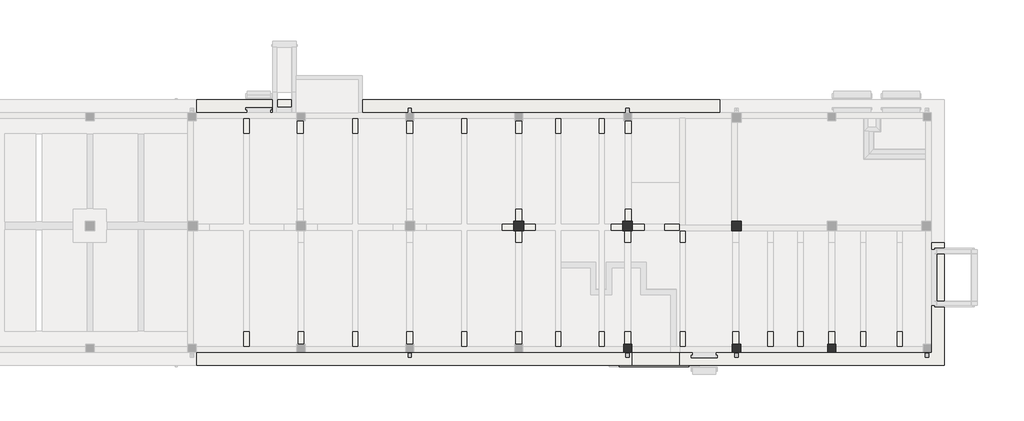
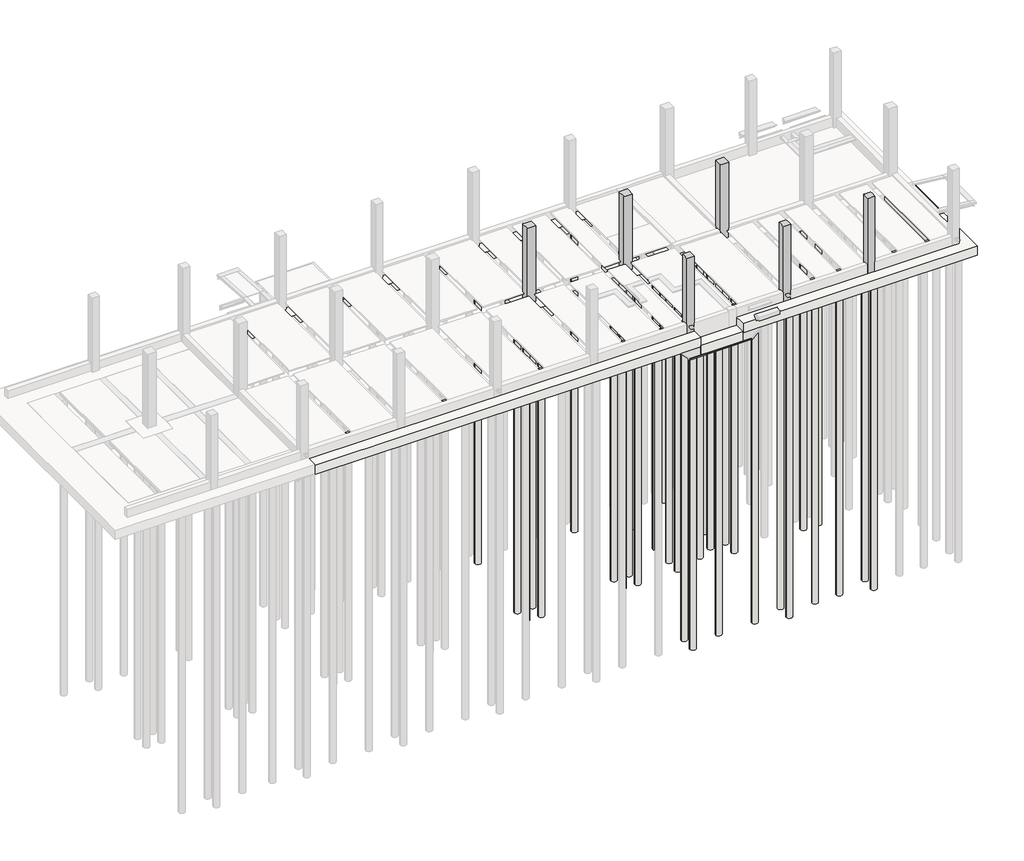
# One storey, part 5 of 7: 42 slabs, 6 columns.
"""IFC4 building model written with IfcOpenShell, lengths in millimetres."""

from ifc_helpers import new_model, si_unit, point, frame, frame_2d, origin, place, context, project, spatial, polyline, circle_curve, trimmed, segment, composite_curve, outline, extrude, faceted_brep, element, save

model = new_model("IFC4")

# Units and contexts
model_context = context("Model", 3, world=origin())
ifc_project = project(units=[si_unit("LENGTHUNIT", "METRE", prefix="MILLI")], contexts=[model_context])

# Site, building, storey
site = spatial("IfcSite", under=ifc_project)
building = spatial("IfcBuilding", under=site)
storey = spatial("IfcBuildingStorey", under=building, Name="H.P.P", Elevation=4500.0)

# Columns
placement = place(None, origin())
element("IfcColumn", 1, ObjectType="RC_Column_Rectangular : H_SC_AR S15_RC Col-AG_700x700_C1", at=placement, inside=storey, context=model_context, shape_type="Brep", body=[
    faceted_brep([(39350.0000001, -7650.0, 4000.0), (39350.0000001, -8350.0, 4000.0), (38650.0000001, -8350.0, 4000.0), (38650.0000001, -7650.0, 4000.0), (39350.0000001, -7650.0, 4650.0), (39350.0000001, -7650.0, 4800.0), (39350.0000001, -7650.0, 10450.0), (39350.0000001, -7650.0, 10600.0), (39350.0000001, -7700.0, 10600.0), (39350.0000001, -8300.0, 10600.0), (39350.0000001, -8350.0, 10600.0), (39350.0000001, -8350.0, 10450.0), (39350.0000001, -8350.0, 4800.0), (39350.0000001, -8350.0, 4650.0), (39249.9999998, -8350.0, 10600.0), (38750.0000002, -8350.0, 10600.0), (38650.0000001, -8350.0, 10600.0), (38650.0000001, -8350.0, 10450.0), (38650.0000001, -8350.0, 4800.0), (38650.0000001, -8350.0, 4650.0), (38650.0000001, -8300.0, 10600.0), (38650.0000001, -7700.0, 10600.0), (38650.0000001, -7650.0, 10600.0), (38650.0000001, -7650.0, 10450.0), (38650.0000001, -7650.0, 4800.0), (38650.0000001, -7650.0, 4650.0), (38750.0000002, -7650.0, 10600.0), (39249.9999998, -7650.0, 10600.0)], [[[0, 1, 2, 3]], [[1, 0, 4, 5, 6, 7, 8, 9, 10, 11, 12, 13]], [[2, 1, 13, 12, 11, 10, 14, 15, 16, 17, 18, 19]], [[3, 2, 19, 18, 17, 16, 20, 21, 22, 23, 24, 25]], [[0, 3, 25, 24, 23, 22, 26, 27, 7, 6, 5, 4]], [[8, 7, 27, 26, 22, 21, 20, 16, 15, 14, 10, 9]]]),
])
element("IfcColumn", 2, ObjectType="RC_Column_Rectangular : H_SC_AR S15_RC Col-AG_700x700_C1", at=placement, inside=storey, context=model_context, shape_type="Brep", body=[
    faceted_brep([(47349.9999999, -7650.0, 4000.0), (47349.9999999, -8350.0, 4000.0), (47250.0, -8350.0, 4000.0), (46750.0, -8350.0, 4000.0), (46649.9999999, -8350.0, 4000.0), (46649.9999999, -7650.0, 4000.0), (47349.9999999, -7650.0, 4650.0), (47349.9999999, -7850.0, 4650.0), (47349.9999999, -7850.0, 4800.0), (47349.9999999, -7650.0, 4800.0), (47349.9999999, -7650.0, 10450.0), (47349.9999999, -7650.0, 10600.0), (47349.9999999, -7750.0, 10600.0), (47349.9999999, -8350.0, 10600.0), (47349.9999999, -8350.0, 10450.0), (47349.9999999, -8350.0, 4800.0), (47349.9999999, -8350.0, 4650.0), (47300.0, -8350.0, 10600.0), (46800.0, -8350.0, 10600.0), (46649.9999999, -8350.0, 10600.0), (46649.9999999, -8350.0, 10450.0), (46649.9999999, -8350.0, 4800.0), (46649.9999999, -8350.0, 4650.0), (46649.9999999, -8300.0, 10600.0), (46649.9999999, -7700.0, 10600.0), (46649.9999999, -7650.0, 10600.0), (46649.9999999, -7650.0, 10450.0), (46649.9999999, -7650.0, 4800.0), (46649.9999999, -7650.0, 4650.0), (46800.0, -7650.0, 10600.0), (47300.0, -7650.0, 10600.0), (47300.0, -7650.0, 4800.0), (47300.0, -7650.0, 4650.0), (47300.0, -7850.0, 4650.0), (47300.0, -7850.0, 4800.0)], [[[0, 1, 2, 3, 4, 5]], [[1, 0, 6, 7, 8, 9, 10, 11, 12, 13, 14, 15, 16]], [[4, 3, 2, 1, 16, 15, 14, 13, 17, 18, 19, 20, 21, 22]], [[5, 4, 22, 21, 20, 19, 23, 24, 25, 26, 27, 28]], [[0, 5, 28, 27, 26, 25, 29, 30, 11, 10, 9, 31, 32, 6]], [[12, 11, 30, 29, 25, 24, 23, 19, 18, 17, 13]], [[32, 33, 7, 6]], [[8, 34, 31, 9]], [[33, 34, 8, 7]], [[34, 33, 32, 31]]]),
])
element("IfcColumn", 3, ObjectType="RC_Column_Rectangular : H_SC_AR S15_RC Col-AG_700x700_C1", at=placement, inside=storey, context=model_context, shape_type="Brep", body=[
    faceted_brep([(55350.0, -7650.0, 4000.0), (55350.0, -7950.0, 4000.0), (55350.0, -8350.0, 4000.0), (54650.0, -8350.0, 4000.0), (54650.0, -7950.0, 4000.0), (54650.0, -7650.0, 4000.0), (55050.0, -7650.0, 4000.0), (55350.0, -7650.0, 10600.0), (55350.0, -8350.0, 10600.0), (55350.0, -8350.0, 10450.0), (55350.0, -8350.0, 9800.0), (55350.0, -8350.0, 4800.0), (55350.0, -8350.0, 4650.0), (55200.0, -8350.0, 10600.0), (54700.0, -8350.0, 10600.0), (54650.0, -8350.0, 10600.0), (54650.0, -8350.0, 10450.0), (54650.0, -8350.0, 9700.0), (54650.0, -8350.0, 4800.0), (54650.0, -8350.0, 4650.0), (54650.0, -7650.0, 10600.0), (54650.0, -7650.0, 9800.0), (54650.0, -7650.0, 4800.0)], [[[0, 1, 2, 3, 4, 5, 6]], [[2, 1, 0, 7, 8, 9, 10, 11, 12]], [[3, 2, 12, 11, 10, 9, 8, 13, 14, 15, 16, 17, 18, 19]], [[5, 4, 3, 19, 18, 17, 16, 15, 20, 21, 22]], [[0, 6, 5, 22, 21, 20, 7]], [[8, 7, 20, 15, 14, 13]]]),
])
element("IfcColumn", 4, ObjectType="RC_Column_Rectangular : H_SC_AR S15_RC Col-AG_600x600_C2", at=placement, inside=storey, context=model_context, shape_type="Brep", body=[
    faceted_brep([(62300.0, -16700.0, 4000.0), (62300.0, -16900.0, 4000.0), (62300.0, -17300.0, 4000.0), (61700.0, -17300.0, 4000.0), (61700.0, -16900.0, 4000.0), (61700.0, -16700.0, 4000.0), (62300.0, -16700.0, 4650.0), (62300.0, -16700.0, 4800.0), (62300.0, -16700.0, 10450.0), (62300.0, -16700.0, 10600.0), (62300.0, -16900.0, 10600.0), (62300.0, -17300.0, 10600.0), (62300.0, -17300.0, 9800.0), (62300.0, -17300.0, 4800.0), (61700.0, -17300.0, 10600.0), (61700.0, -17300.0, 9800.0), (61700.0, -17300.0, 4800.0), (61700.0, -16900.0, 10600.0), (61700.0, -16700.0, 10600.0), (61700.0, -16700.0, 10450.0), (61700.0, -16700.0, 4800.0), (61700.0, -16700.0, 4650.0), (61750.0, -16700.0, 10600.0), (62250.0, -16700.0, 10600.0)], [[[0, 1, 2, 3, 4, 5]], [[2, 1, 0, 6, 7, 8, 9, 10, 11, 12, 13]], [[3, 2, 13, 12, 11, 14, 15, 16]], [[5, 4, 3, 16, 15, 14, 17, 18, 19, 20, 21]], [[0, 5, 21, 20, 19, 18, 22, 23, 9, 8, 7, 6]], [[14, 11, 10, 9, 23, 22, 18, 17]]]),
])
element("IfcColumn", 5, ObjectType="RC_Column_Rectangular : H_SC_AR S15_RC Col-AG_600x600_C2", at=placement, inside=storey, context=model_context, shape_type="Brep", body=[
    faceted_brep([(55300.0, -16700.0, 4000.0), (55300.0, -16900.0, 4000.0), (55300.0, -17300.0, 4000.0), (54700.0, -17300.0, 4000.0), (54700.0, -16900.0, 4000.0), (54700.0, -16700.0, 4000.0), (55300.0, -16700.0, 4650.0), (55300.0, -16700.0, 4800.0), (55300.0, -16700.0, 10450.0), (55300.0, -16700.0, 10600.0), (55300.0, -16900.0, 10600.0), (55300.0, -17300.0, 10600.0), (55300.0, -17300.0, 9800.0), (55300.0, -17300.0, 4800.0), (54700.0, -17300.0, 10600.0), (54700.0, -17300.0, 9800.0), (54700.0, -17300.0, 4800.0), (54700.0, -16900.0, 10600.0), (54700.0, -16700.0, 10600.0), (54700.0, -16700.0, 10450.0), (54700.0, -16700.0, 4800.0), (54700.0, -16700.0, 4650.0), (55200.0, -16700.0, 10600.0)], [[[0, 1, 2, 3, 4, 5]], [[2, 1, 0, 6, 7, 8, 9, 10, 11, 12, 13]], [[3, 2, 13, 12, 11, 14, 15, 16]], [[5, 4, 3, 16, 15, 14, 17, 18, 19, 20, 21]], [[0, 5, 21, 20, 19, 18, 22, 9, 8, 7, 6]], [[14, 11, 10, 9, 22, 18, 17]]]),
])
element("IfcColumn", 6, ObjectType="RC_Column_Rectangular : H_SC_AR S15_RC Col-AG_600x600_C2", at=placement, inside=storey, context=model_context, shape_type="Brep", body=[
    faceted_brep([(46700.0, -16700.0, 4000.0), (47300.0, -16700.0, 4000.0), (47300.0, -17300.0, 4000.0), (46700.0, -17300.0, 4000.0), (46700.0, -16900.0, 4000.0), (46700.0, -16700.0, 4550.0), (46700.0, -16700.0, 4700.0), (46700.0, -16700.0, 10450.0), (46700.0, -16700.0, 10600.0), (46800.0, -16700.0, 10600.0), (47300.0, -16700.0, 10600.0), (47300.0, -16700.0, 10450.0), (47300.0, -16700.0, 4700.0), (47300.0, -16700.0, 4550.0), (47300.0, -16900.0, 10600.0), (47300.0, -17300.0, 10600.0), (47300.0, -17300.0, 9800.0), (47300.0, -17300.0, 4700.0), (46700.0, -17300.0, 10600.0), (46700.0, -17300.0, 9800.0), (46700.0, -17300.0, 4800.0), (46700.0, -16900.0, 10600.0)], [[[0, 1, 2, 3, 4]], [[1, 0, 5, 6, 7, 8, 9, 10, 11, 12, 13]], [[2, 1, 13, 12, 11, 10, 14, 15, 16, 17]], [[3, 2, 17, 16, 15, 18, 19, 20]], [[0, 4, 3, 20, 19, 18, 21, 8, 7, 6, 5]], [[18, 15, 14, 10, 9, 8, 21]]]),
])

# Slabs
element("IfcSlab", 7, ObjectType="H_SF_AR S18_MAT_T800_WF1", at=placement, inside=storey, context=model_context, shape_type="Brep", body=[
    faceted_brep([(50825.0, -18250.0000001, 3200.0), (50825.0, -15750.0000001, 3200.0), (52225.0, -15750.0000001, 3200.0), (67750.0000002, -15750.0000001, 3200.0), (67750.0000002, -9250.0, 3200.0), (70250.0, -9250.0, 3200.0), (70250.0, -18250.0000001, 3200.0), (52225.0, -18250.0000001, 3200.0), (50825.0, -18250.0000001, 4000.0), (70250.0, -18250.0000001, 4000.0), (70250.0, -9250.0, 4000.0), (67750.0000002, -9250.0, 4000.0), (67750.0000002, -15750.0000001, 4000.0), (50825.0, -15750.0000001, 4000.0), (50825.0, -16900.0, 4000.0), (50825.0, -18250.0000001, 3300.0), (50825.0, -15750.0000001, 3300.0)], [[[0, 1, 2, 3, 4, 5, 6, 7]], [[8, 9, 10, 11, 12, 13, 14]], [[6, 5, 10, 9]], [[0, 7, 6, 9, 8, 15]], [[3, 2, 1, 16, 13, 12]], [[4, 3, 12, 11]], [[1, 0, 15, 8, 14, 13, 16]], [[5, 4, 11, 10]]]),
    faceted_brep([(15299.9999999, -18250.0000001, 3200.0), (15299.9999999, -15750.0000001, 3200.0), (45675.0, -15750.0000001, 3200.0), (47300.0, -15750.0000001, 3200.0), (47300.0, -18250.0000001, 3200.0), (45675.0, -18250.0000001, 3200.0), (15299.9999999, -18250.0000001, 4000.0), (47300.0, -18250.0000001, 4000.0), (47300.0, -15750.0000001, 4000.0), (15299.9999999, -15750.0000001, 4000.0), (15299.9999999, -18250.0000001, 3300.0), (15299.9999999, -15750.0000001, 3300.0), (47300.0, -15750.0000001, 3300.0), (47300.0, -18250.0000001, 3300.0)], [[[0, 1, 2, 3, 4, 5]], [[6, 7, 8, 9]], [[1, 0, 10, 6, 9, 11]], [[3, 2, 1, 11, 9, 8, 12]], [[4, 3, 12, 8, 7, 13]], [[0, 5, 4, 13, 7, 6, 10]]]),
    faceted_brep([(53749.9998007, 1249.9999999, 3200.0), (53749.9998007, -1250.0000001, 3200.0), (52200.0000002, -1250.0000001, 3200.0), (52200.0000002, -6750.0000001, 3200.0), (53749.9998007, -6750.0000001, 3200.0), (53749.9998007, -9250.0, 3200.0), (49700.0000002, -9250.0, 3200.0), (49700.0000002, -1250.0000001, 3200.0), (15299.9999999, -1250.0000001, 3200.0), (15299.9999999, 1249.9999999, 3200.0), (53749.9998007, 1249.9999999, 4000.0), (15299.9999999, 1249.9999999, 4000.0), (15299.9999999, -1250.0000001, 4000.0), (49700.0000002, -1250.0000001, 4000.0), (49700.0000002, -9250.0, 4000.0), (53749.9998007, -9250.0, 4000.0), (53749.9998007, -6750.0000001, 4000.0), (52200.0000002, -6750.0000001, 4000.0), (52200.0000002, -1250.0000001, 4000.0), (53749.9998007, -1250.0000001, 4000.0), (15299.9999999, 1249.9999999, 3300.0), (15299.9999999, -1250.0000001, 3300.0)], [[[0, 1, 2, 3, 4, 5, 6, 7, 8, 9]], [[10, 11, 12, 13, 14, 15, 16, 17, 18, 19]], [[0, 9, 20, 11, 10]], [[6, 5, 15, 14]], [[7, 6, 14, 13]], [[8, 7, 13, 12, 21]], [[2, 1, 19, 18]], [[3, 2, 18, 17]], [[4, 3, 17, 16]], [[1, 0, 10, 19]], [[9, 8, 21, 12, 11, 20]], [[5, 4, 16, 15]]]),
])
element("IfcSlab", 8, ObjectType="H_SF_AR S18_MAT_T800_WF1", at=placement, inside=storey, context=model_context, shape_type="Brep", body=[
    faceted_brep([(50825.0, -15750.0000001, 2500.0), (50825.0, -18250.0000001, 2500.0), (47300.0, -18250.0000001, 2500.0), (47300.0, -15750.0000001, 2500.0), (50825.0, -18250.0000001, 3300.0), (50825.0, -15750.0000001, 3300.0), (47300.0, -15750.0000001, 3300.0), (47300.0, -18250.0000001, 3300.0), (50825.0, -15750.0000001, 3200.0), (50825.0, -18250.0000001, 3200.0), (47300.0, -18250.0000001, 3200.0), (47300.0, -15750.0000001, 3200.0)], [[[0, 1, 2, 3]], [[4, 5, 6, 7]], [[1, 0, 8, 5, 4, 9]], [[2, 1, 9, 4, 7, 10]], [[3, 2, 10, 7, 6, 11]], [[0, 3, 11, 6, 5, 8]]]),
])
element("IfcSlab", 9, ObjectType="H_SF_AR_S18_Lean_T50", at=placement, inside=storey, context=model_context, shape_type="SweptSolid", body=[
    extrude(outline(polyline([(51525.0, -15650.0), (51525.0, -18350.0000001), (46375.0, -18350.0000001), (46375.0, -15650.0), (51525.0, -15650.0)])), frame((0.0, 0.0, 2450.0), z_axis=(0.0, 0.0, 1.0), x_axis=(1.0, 0.0, 0.0)), (0.0, 0.0, 1.0), 50.0),
])
element("IfcSlab", 10, ObjectType="H_SF_AR_S18_Lean_T50", at=placement, inside=storey, context=model_context, shape_type="Brep", body=[
    faceted_brep([(50475.0, -16790.0, 4390.0), (47360.0, -16790.0, 4390.0), (47360.0, -10775.0, 4390.0), (48275.0, -10775.0, 4390.0), (48275.0, -12775.0, 4390.0), (50475.0, -12775.0, 4390.0), (47360.0, -16790.0, 4440.0), (50475.0, -16790.0, 4440.0), (50475.0, -12775.0, 4440.0), (48275.0, -12775.0, 4440.0), (48275.0, -10775.0, 4440.0), (47360.0, -10775.0, 4440.0)], [[[0, 1, 2, 3, 4, 5]], [[6, 7, 8, 9, 10, 11]], [[1, 0, 7, 6]], [[2, 1, 6, 11]], [[3, 2, 11, 10]], [[4, 3, 10, 9]], [[5, 4, 9, 8]], [[0, 5, 8, 7]]]),
    faceted_brep([(46640.0, -10775.0, 4390.0), (46640.0, -16790.0, 4390.0), (45435.0, -16790.0, 4390.0), (45435.0, -12775.0, 4390.0), (45504.2893219, -12775.0, 4390.0), (45525.0, -12775.0, 4390.0), (45525.0, -10775.0, 4390.0), (46640.0, -16790.0, 4440.0), (46640.0, -10775.0, 4440.0), (45525.0, -10775.0, 4440.0), (45525.0, -12775.0, 4440.0), (45454.2893219, -12775.0, 4440.0), (45435.0, -12775.0, 4440.0), (45435.0, -16790.0, 4440.0)], [[[0, 1, 2, 3, 4, 5, 6]], [[7, 8, 9, 10, 11, 12, 13]], [[1, 0, 8, 7]], [[2, 1, 7, 13]], [[3, 2, 13, 12]], [[3, 12, 11, 10, 5, 4]], [[6, 5, 10, 9]], [[0, 6, 9, 8]]]),
    faceted_brep([(44765.0, -12775.0, 4390.0), (44765.0, -16790.0, 4390.0), (42235.0, -16790.0, 4390.0), (42235.0, -10775.0, 4390.0), (44575.0, -10775.0, 4390.0), (44575.0, -12775.0, 4390.0), (44765.0, -16790.0, 4440.0), (44765.0, -12775.0, 4440.0), (44575.0, -12775.0, 4440.0), (44575.0, -10775.0, 4440.0), (42235.0, -10775.0, 4440.0), (42235.0, -16790.0, 4440.0)], [[[0, 1, 2, 3, 4, 5]], [[6, 7, 8, 9, 10, 11]], [[1, 0, 7, 6]], [[2, 1, 6, 11]], [[3, 2, 11, 10]], [[4, 3, 10, 9]], [[5, 4, 9, 8]], [[0, 5, 8, 7]]]),
    faceted_brep([(47410.0, -4825.0, 4390.0), (47410.0, -210.0, 4390.0), (50825.0, -210.0, 4390.0), (50825.0, -4825.0, 4390.0), (47410.0, -210.0, 4440.0), (47410.0, -4825.0, 4440.0), (50825.0, -4825.0, 4440.0), (50825.0, -210.0, 4440.0)], [[[0, 1, 2, 3]], [[4, 5, 6, 7]], [[1, 0, 5, 4]], [[2, 1, 4, 7]], [[3, 2, 7, 6]], [[0, 3, 6, 5]]]),
])
element("IfcSlab", 11, ObjectType="H_SF_AR_S18_Lean_T50", at=placement, inside=storey, context=model_context, shape_type="SweptSolid", body=[
    extrude(outline(polyline([(54650.0, -100.0), (54650.0, -7950.0), (51225.0, -7950.0), (51225.0, -100.0), (54650.0, -100.0)])), frame((0.0, 0.0, 4440.0), z_axis=(0.0, 0.0, 1.0), x_axis=(1.0, 0.0, 0.0)), (0.0, 0.0, 1.0), 50.0),
])
element("IfcSlab", 12, ObjectType="Foundation Rectangular (Non-Pile) : H_SF_AR S18_Ret Fdn_2500x2500xT1000_F1A", at=placement, inside=storey, context=model_context, shape_type="SweptSolid", body=[
    extrude(outline(polyline([(40250.0000001, -6750.0), (40250.0000001, -9250.0), (37750.0000001, -9250.0), (37750.0000001, -6750.0), (40250.0000001, -6750.0)])), frame((0.0, 0.0, 3000.0), z_axis=(0.0, 0.0, 1.0), x_axis=(1.0, 0.0, 0.0)), (0.0, 0.0, 1.0), 1000.0),
])
element("IfcSlab", 13, ObjectType="Foundation Rectangular (Non-Pile) : H_SF_AR S18_Ret Fdn_2500x2500xT1000_F1A", at=placement, inside=storey, context=model_context, shape_type="SweptSolid", body=[
    extrude(outline(polyline([(48249.9999999, -6750.0), (48249.9999999, -9250.0), (45749.9999999, -9250.0), (45749.9999999, -6750.0), (48249.9999999, -6750.0)])), frame((0.0, 0.0, 3000.0), z_axis=(0.0, 0.0, 1.0), x_axis=(1.0, 0.0, 0.0)), (0.0, 0.0, 1.0), 1000.0),
])
element("IfcSlab", 14, ObjectType="PILE : H_FL_AR S19_Pile_D500_L26.8", at=placement, inside=storey, context=model_context, shape_type="SweptSolid", body=[
    extrude(outline(composite_curve([segment(trimmed(circle_curve(frame_2d((39000.0, -625.0)), 250.0), [point((38750.0, -625.0))], [point((39250.0, -625.0))], False, "CARTESIAN"), True, "CONTINUOUS"), segment(trimmed(circle_curve(frame_2d((39000.0, -625.0)), 250.0), [point((39250.0, -625.0))], [point((38750.0, -625.0))], False, "CARTESIAN"), True, "CONTINUOUS")], self_intersect=False)), frame((0.0, 0.0, -23500.0), z_axis=(0.0, 0.0, 1.0), x_axis=(1.0, 0.0, 0.0)), (0.0, 0.0, 1.0), 26650.0),
])
element("IfcSlab", 15, ObjectType="PILE : H_FL_AR S19_Pile_D500_L26.8", at=placement, inside=storey, context=model_context, shape_type="SweptSolid", body=[
    extrude(outline(composite_curve([segment(trimmed(circle_curve(frame_2d((47000.0, -625.0000002)), 250.0), [point((46750.0, -625.0000002))], [point((47250.0, -625.0000002))], False, "CARTESIAN"), True, "CONTINUOUS"), segment(trimmed(circle_curve(frame_2d((47000.0, -625.0000002)), 250.0), [point((47250.0, -625.0000002))], [point((46750.0, -625.0000002))], False, "CARTESIAN"), True, "CONTINUOUS")], self_intersect=False)), frame((0.0, 0.0, -23500.0), z_axis=(0.0, 0.0, 1.0), x_axis=(1.0, 0.0, 0.0)), (0.0, 0.0, 1.0), 26650.0),
])
element("IfcSlab", 16, ObjectType="PILE : H_FL_AR S19_Pile_D500_L26.8", at=placement, inside=storey, context=model_context, shape_type="SweptSolid", body=[
    extrude(outline(composite_curve([segment(trimmed(circle_curve(frame_2d((50950.0000002, -625.0)), 250.0), [point((50700.0000002, -625.0))], [point((51200.0000002, -625.0))], False, "CARTESIAN"), True, "CONTINUOUS"), segment(trimmed(circle_curve(frame_2d((50950.0000002, -625.0)), 250.0), [point((51200.0000002, -625.0))], [point((50700.0000002, -625.0))], False, "CARTESIAN"), True, "CONTINUOUS")], self_intersect=False)), frame((0.0, 0.0, -23500.0), z_axis=(0.0, 0.0, 1.0), x_axis=(1.0, 0.0, 0.0)), (0.0, 0.0, 1.0), 26650.0),
])
element("IfcSlab", 17, ObjectType="PILE : H_FL_AR S19_Pile_D500_L26.8", at=placement, inside=storey, context=model_context, shape_type="SweptSolid", body=[
    extrude(outline(composite_curve([segment(trimmed(circle_curve(frame_2d((50950.0000002, -2500.0)), 250.0), [point((50700.0000002, -2500.0))], [point((51200.0000002, -2500.0))], False, "CARTESIAN"), True, "CONTINUOUS"), segment(trimmed(circle_curve(frame_2d((50950.0000002, -2500.0)), 250.0), [point((51200.0000002, -2500.0))], [point((50700.0000002, -2500.0))], False, "CARTESIAN"), True, "CONTINUOUS")], self_intersect=False)), frame((0.0, 0.0, -23500.0), z_axis=(0.0, 0.0, 1.0), x_axis=(1.0, 0.0, 0.0)), (0.0, 0.0, 1.0), 26650.0),
])
element("IfcSlab", 18, ObjectType="PILE : H_FL_AR S19_Pile_D500_L26.8", at=placement, inside=storey, context=model_context, shape_type="SweptSolid", body=[
    extrude(outline(composite_curve([segment(trimmed(circle_curve(frame_2d((50950.0000002, -5500.0)), 250.0), [point((50700.0000002, -5500.0))], [point((51200.0000002, -5500.0))], False, "CARTESIAN"), True, "CONTINUOUS"), segment(trimmed(circle_curve(frame_2d((50950.0000002, -5500.0)), 250.0), [point((51200.0000002, -5500.0))], [point((50700.0000002, -5500.0))], False, "CARTESIAN"), True, "CONTINUOUS")], self_intersect=False)), frame((0.0, 0.0, -23500.0), z_axis=(0.0, 0.0, 1.0), x_axis=(1.0, 0.0, 0.0)), (0.0, 0.0, 1.0), 26650.0),
])
element("IfcSlab", 19, ObjectType="PILE : H_FL_AR S19_Pile_D500_L26.8", at=placement, inside=storey, context=model_context, shape_type="SweptSolid", body=[
    extrude(outline(composite_curve([segment(trimmed(circle_curve(frame_2d((50950.0000002, -7375.0000222)), 250.0), [point((50700.0000002, -7375.0000222))], [point((51200.0000002, -7375.0000222))], False, "CARTESIAN"), True, "CONTINUOUS"), segment(trimmed(circle_curve(frame_2d((50950.0000002, -7375.0000222)), 250.0), [point((51200.0000002, -7375.0000222))], [point((50700.0000002, -7375.0000222))], False, "CARTESIAN"), True, "CONTINUOUS")], self_intersect=False)), frame((0.0, 0.0, -23500.0), z_axis=(0.0, 0.0, 1.0), x_axis=(1.0, 0.0, 0.0)), (0.0, 0.0, 1.0), 26650.0),
])
element("IfcSlab", 20, ObjectType="PILE : H_FL_AR S19_Pile_D500_L26.8", at=placement, inside=storey, context=model_context, shape_type="SweptSolid", body=[
    extrude(outline(composite_curve([segment(trimmed(circle_curve(frame_2d((50950.0000002, -8625.0000222)), 250.0), [point((50700.0000002, -8625.0000222))], [point((51200.0000002, -8625.0000222))], False, "CARTESIAN"), True, "CONTINUOUS"), segment(trimmed(circle_curve(frame_2d((50950.0000002, -8625.0000222)), 250.0), [point((51200.0000002, -8625.0000222))], [point((50700.0000002, -8625.0000222))], False, "CARTESIAN"), True, "CONTINUOUS")], self_intersect=False)), frame((0.0, 0.0, -23500.0), z_axis=(0.0, 0.0, 1.0), x_axis=(1.0, 0.0, 0.0)), (0.0, 0.0, 1.0), 26650.0),
])
element("IfcSlab", 21, ObjectType="PILE : H_FL_AR S19_Pile_D500_L26.8", at=placement, inside=storey, context=model_context, shape_type="SweptSolid", body=[
    extrude(outline(composite_curve([segment(trimmed(circle_curve(frame_2d((53125.0, -8000.0)), 250.0), [point((52875.0, -8000.0))], [point((53375.0, -8000.0))], False, "CARTESIAN"), True, "CONTINUOUS"), segment(trimmed(circle_curve(frame_2d((53125.0, -8000.0)), 250.0), [point((53375.0, -8000.0))], [point((52875.0, -8000.0))], False, "CARTESIAN"), True, "CONTINUOUS")], self_intersect=False)), frame((0.0, 0.0, -23500.0), z_axis=(0.0, 0.0, 1.0), x_axis=(1.0, 0.0, 0.0)), (0.0, 0.0, 1.0), 26650.0),
])
element("IfcSlab", 22, ObjectType="PILE : H_FL_AR S19_Pile_D500_L26.6", at=placement, inside=storey, context=model_context, shape_type="SweptSolid", body=[
    extrude(outline(composite_curve([segment(trimmed(circle_curve(frame_2d((38375.0000004, -7374.9999999)), 250.0), [point((38125.0000004, -7374.9999999))], [point((38625.0000004, -7374.9999999))], False, "CARTESIAN"), True, "CONTINUOUS"), segment(trimmed(circle_curve(frame_2d((38375.0000004, -7374.9999999)), 250.0), [point((38625.0000004, -7374.9999999))], [point((38125.0000004, -7374.9999999))], False, "CARTESIAN"), True, "CONTINUOUS")], self_intersect=False)), frame((0.0, 0.0, -23500.0), z_axis=(0.0, 0.0, 1.0), x_axis=(1.0, 0.0, 0.0)), (0.0, 0.0, 1.0), 26450.0),
])
element("IfcSlab", 23, ObjectType="PILE : H_FL_AR S19_Pile_D500_L26.6", at=placement, inside=storey, context=model_context, shape_type="SweptSolid", body=[
    extrude(outline(composite_curve([segment(trimmed(circle_curve(frame_2d((39625.0000004, -7374.9999999)), 250.0), [point((39375.0000004, -7374.9999999))], [point((39875.0000004, -7374.9999999))], False, "CARTESIAN"), True, "CONTINUOUS"), segment(trimmed(circle_curve(frame_2d((39625.0000004, -7374.9999999)), 250.0), [point((39875.0000004, -7374.9999999))], [point((39375.0000004, -7374.9999999))], False, "CARTESIAN"), True, "CONTINUOUS")], self_intersect=False)), frame((0.0, 0.0, -23500.0), z_axis=(0.0, 0.0, 1.0), x_axis=(1.0, 0.0, 0.0)), (0.0, 0.0, 1.0), 26450.0),
])
element("IfcSlab", 24, ObjectType="PILE : H_FL_AR S19_Pile_D500_L26.6", at=placement, inside=storey, context=model_context, shape_type="SweptSolid", body=[
    extrude(outline(composite_curve([segment(trimmed(circle_curve(frame_2d((38375.0000004, -8624.9999999)), 250.0), [point((38125.0000004, -8624.9999999))], [point((38625.0000004, -8624.9999999))], False, "CARTESIAN"), True, "CONTINUOUS"), segment(trimmed(circle_curve(frame_2d((38375.0000004, -8624.9999999)), 250.0), [point((38625.0000004, -8624.9999999))], [point((38125.0000004, -8624.9999999))], False, "CARTESIAN"), True, "CONTINUOUS")], self_intersect=False)), frame((0.0, 0.0, -23500.0), z_axis=(0.0, 0.0, 1.0), x_axis=(1.0, 0.0, 0.0)), (0.0, 0.0, 1.0), 26450.0),
])
element("IfcSlab", 25, ObjectType="PILE : H_FL_AR S19_Pile_D500_L26.6", at=placement, inside=storey, context=model_context, shape_type="SweptSolid", body=[
    extrude(outline(composite_curve([segment(trimmed(circle_curve(frame_2d((39625.0000004, -8624.9999999)), 250.0), [point((39375.0000004, -8624.9999999))], [point((39875.0000004, -8624.9999999))], False, "CARTESIAN"), True, "CONTINUOUS"), segment(trimmed(circle_curve(frame_2d((39625.0000004, -8624.9999999)), 250.0), [point((39875.0000004, -8624.9999999))], [point((39375.0000004, -8624.9999999))], False, "CARTESIAN"), True, "CONTINUOUS")], self_intersect=False)), frame((0.0, 0.0, -23500.0), z_axis=(0.0, 0.0, 1.0), x_axis=(1.0, 0.0, 0.0)), (0.0, 0.0, 1.0), 26450.0),
])
element("IfcSlab", 26, ObjectType="PILE : H_FL_AR S19_Pile_D500_L26.6", at=placement, inside=storey, context=model_context, shape_type="SweptSolid", body=[
    extrude(outline(composite_curve([segment(trimmed(circle_curve(frame_2d((46375.0000004, -7374.9999999)), 250.0), [point((46125.0000004, -7374.9999999))], [point((46625.0000004, -7374.9999999))], False, "CARTESIAN"), True, "CONTINUOUS"), segment(trimmed(circle_curve(frame_2d((46375.0000004, -7374.9999999)), 250.0), [point((46625.0000004, -7374.9999999))], [point((46125.0000004, -7374.9999999))], False, "CARTESIAN"), True, "CONTINUOUS")], self_intersect=False)), frame((0.0, 0.0, -23500.0), z_axis=(0.0, 0.0, 1.0), x_axis=(1.0, 0.0, 0.0)), (0.0, 0.0, 1.0), 26450.0),
])
element("IfcSlab", 27, ObjectType="PILE : H_FL_AR S19_Pile_D500_L26.6", at=placement, inside=storey, context=model_context, shape_type="SweptSolid", body=[
    extrude(outline(composite_curve([segment(trimmed(circle_curve(frame_2d((47625.0000004, -7374.9999999)), 250.0), [point((47375.0000004, -7374.9999999))], [point((47875.0000004, -7374.9999999))], False, "CARTESIAN"), True, "CONTINUOUS"), segment(trimmed(circle_curve(frame_2d((47625.0000004, -7374.9999999)), 250.0), [point((47875.0000004, -7374.9999999))], [point((47375.0000004, -7374.9999999))], False, "CARTESIAN"), True, "CONTINUOUS")], self_intersect=False)), frame((0.0, 0.0, -23500.0), z_axis=(0.0, 0.0, 1.0), x_axis=(1.0, 0.0, 0.0)), (0.0, 0.0, 1.0), 26450.0),
])
element("IfcSlab", 28, ObjectType="PILE : H_FL_AR S19_Pile_D500_L26.6", at=placement, inside=storey, context=model_context, shape_type="SweptSolid", body=[
    extrude(outline(composite_curve([segment(trimmed(circle_curve(frame_2d((46375.0000004, -8624.9999999)), 250.0), [point((46125.0000004, -8624.9999999))], [point((46625.0000004, -8624.9999999))], False, "CARTESIAN"), True, "CONTINUOUS"), segment(trimmed(circle_curve(frame_2d((46375.0000004, -8624.9999999)), 250.0), [point((46625.0000004, -8624.9999999))], [point((46125.0000004, -8624.9999999))], False, "CARTESIAN"), True, "CONTINUOUS")], self_intersect=False)), frame((0.0, 0.0, -23500.0), z_axis=(0.0, 0.0, 1.0), x_axis=(1.0, 0.0, 0.0)), (0.0, 0.0, 1.0), 26450.0),
])
element("IfcSlab", 29, ObjectType="PILE : H_FL_AR S19_Pile_D500_L26.6", at=placement, inside=storey, context=model_context, shape_type="SweptSolid", body=[
    extrude(outline(composite_curve([segment(trimmed(circle_curve(frame_2d((47625.0000004, -8624.9999999)), 250.0), [point((47375.0000004, -8624.9999999))], [point((47875.0000004, -8624.9999999))], False, "CARTESIAN"), True, "CONTINUOUS"), segment(trimmed(circle_curve(frame_2d((47625.0000004, -8624.9999999)), 250.0), [point((47875.0000004, -8624.9999999))], [point((47375.0000004, -8624.9999999))], False, "CARTESIAN"), True, "CONTINUOUS")], self_intersect=False)), frame((0.0, 0.0, -23500.0), z_axis=(0.0, 0.0, 1.0), x_axis=(1.0, 0.0, 0.0)), (0.0, 0.0, 1.0), 26450.0),
])
element("IfcSlab", 30, ObjectType="PILE : H_FL_AR S19_Pile_D500_L26.1", at=placement, inside=storey, context=model_context, shape_type="SweptSolid", body=[
    extrude(outline(composite_curve([segment(trimmed(circle_curve(frame_2d((47000.0, -16375.0000002)), 250.0), [point((47250.0, -16375.0000002))], [point((46750.0, -16375.0000002))], False, "CARTESIAN"), True, "CONTINUOUS"), segment(trimmed(circle_curve(frame_2d((47000.0, -16375.0000002)), 250.0), [point((46750.0, -16375.0000002))], [point((47250.0, -16375.0000002))], False, "CARTESIAN"), True, "CONTINUOUS")], self_intersect=False)), frame((0.0, 0.0, 2500.0), z_axis=(0.0, 0.0, 1.0), x_axis=(1.0, 0.0, 0.0)), (0.0, 0.0, 1.0), 100.0),
    extrude(outline(composite_curve([segment(trimmed(circle_curve(frame_2d((47000.0, -16375.0000002)), 250.0), [point((46750.0, -16375.0000002))], [point((47250.0, -16375.0000002))], False, "CARTESIAN"), True, "CONTINUOUS"), segment(trimmed(circle_curve(frame_2d((47000.0, -16375.0000002)), 250.0), [point((47250.0, -16375.0000002))], [point((46750.0, -16375.0000002))], False, "CARTESIAN"), True, "CONTINUOUS")], self_intersect=False)), frame((0.0, 0.0, -23500.0), z_axis=(0.0, 0.0, 1.0), x_axis=(1.0, 0.0, 0.0)), (0.0, 0.0, 1.0), 25950.0),
])
element("IfcSlab", 31, ObjectType="PILE : H_FL_AR S19_Pile_D500_L26.1", at=placement, inside=storey, context=model_context, shape_type="SweptSolid", body=[
    extrude(outline(composite_curve([segment(trimmed(circle_curve(frame_2d((47000.0, -17624.9999997)), 250.0), [point((47250.0, -17624.9999997))], [point((46750.0, -17624.9999997))], False, "CARTESIAN"), True, "CONTINUOUS"), segment(trimmed(circle_curve(frame_2d((47000.0, -17624.9999997)), 250.0), [point((46750.0, -17624.9999997))], [point((47250.0, -17624.9999997))], False, "CARTESIAN"), True, "CONTINUOUS")], self_intersect=False)), frame((0.0, 0.0, 2500.0), z_axis=(0.0, 0.0, 1.0), x_axis=(1.0, 0.0, 0.0)), (0.0, 0.0, 1.0), 100.0),
    extrude(outline(composite_curve([segment(trimmed(circle_curve(frame_2d((47000.0, -17624.9999997)), 250.0), [point((46750.0, -17624.9999997))], [point((47250.0, -17624.9999997))], False, "CARTESIAN"), True, "CONTINUOUS"), segment(trimmed(circle_curve(frame_2d((47000.0, -17624.9999997)), 250.0), [point((47250.0, -17624.9999997))], [point((46750.0, -17624.9999997))], False, "CARTESIAN"), True, "CONTINUOUS")], self_intersect=False)), frame((0.0, 0.0, -23500.0), z_axis=(0.0, 0.0, 1.0), x_axis=(1.0, 0.0, 0.0)), (0.0, 0.0, 1.0), 25950.0),
])
element("IfcSlab", 32, ObjectType="PILE : H_FL_AR S19_Pile_D500_L26.1", at=placement, inside=storey, context=model_context, shape_type="SweptSolid", body=[
    extrude(outline(composite_curve([segment(trimmed(circle_curve(frame_2d((49500.0000012, -17000.0)), 250.0), [point((49250.0000012, -17000.0))], [point((49750.0000012, -17000.0))], False, "CARTESIAN"), True, "CONTINUOUS"), segment(trimmed(circle_curve(frame_2d((49500.0000012, -17000.0)), 250.0), [point((49750.0000012, -17000.0))], [point((49250.0000012, -17000.0))], False, "CARTESIAN"), True, "CONTINUOUS")], self_intersect=False)), frame((0.0, 0.0, -23500.0), z_axis=(0.0, 0.0, 1.0), x_axis=(1.0, 0.0, 0.0)), (0.0, 0.0, 1.0), 25950.0),
])
element("IfcSlab", 33, ObjectType="PILE : H_FL_AR S19_Pile_D500_L26.8", at=placement, inside=storey, context=model_context, shape_type="SweptSolid", body=[
    extrude(outline(composite_curve([segment(trimmed(circle_curve(frame_2d((52500.0000003, -17000.0)), 250.0), [point((52250.0000003, -17000.0))], [point((52750.0000003, -17000.0))], False, "CARTESIAN"), True, "CONTINUOUS"), segment(trimmed(circle_curve(frame_2d((52500.0000003, -17000.0)), 250.0), [point((52750.0000003, -17000.0))], [point((52250.0000003, -17000.0))], False, "CARTESIAN"), True, "CONTINUOUS")], self_intersect=False)), frame((0.0, 0.0, -23500.0), z_axis=(0.0, 0.0, 1.0), x_axis=(1.0, 0.0, 0.0)), (0.0, 0.0, 1.0), 26650.0),
])
element("IfcSlab", 34, ObjectType="PILE : H_FL_AR S19_Pile_D500_L26.8", at=placement, inside=storey, context=model_context, shape_type="SweptSolid", body=[
    extrude(outline(composite_curve([segment(trimmed(circle_curve(frame_2d((55000.0, -16375.0000004)), 250.0), [point((54750.0, -16375.0000004))], [point((55250.0, -16375.0000004))], False, "CARTESIAN"), True, "CONTINUOUS"), segment(trimmed(circle_curve(frame_2d((55000.0, -16375.0000004)), 250.0), [point((55250.0, -16375.0000004))], [point((54750.0, -16375.0000004))], False, "CARTESIAN"), True, "CONTINUOUS")], self_intersect=False)), frame((0.0, 0.0, -23500.0), z_axis=(0.0, 0.0, 1.0), x_axis=(1.0, 0.0, 0.0)), (0.0, 0.0, 1.0), 26650.0),
])
element("IfcSlab", 35, ObjectType="PILE : H_FL_AR S19_Pile_D500_L26.8", at=placement, inside=storey, context=model_context, shape_type="SweptSolid", body=[
    extrude(outline(composite_curve([segment(trimmed(circle_curve(frame_2d((55000.0, -17625.0)), 250.0), [point((54750.0, -17625.0))], [point((55250.0, -17625.0))], False, "CARTESIAN"), True, "CONTINUOUS"), segment(trimmed(circle_curve(frame_2d((55000.0, -17625.0)), 250.0), [point((55250.0, -17625.0))], [point((54750.0, -17625.0))], False, "CARTESIAN"), True, "CONTINUOUS")], self_intersect=False)), frame((0.0, 0.0, -23500.0), z_axis=(0.0, 0.0, 1.0), x_axis=(1.0, 0.0, 0.0)), (0.0, 0.0, 1.0), 26650.0),
])
element("IfcSlab", 36, ObjectType="PILE : H_FL_AR S19_Pile_D500_L26.8", at=placement, inside=storey, context=model_context, shape_type="SweptSolid", body=[
    extrude(outline(composite_curve([segment(trimmed(circle_curve(frame_2d((57499.9999998, -17000.0)), 250.0), [point((57249.9999998, -17000.0))], [point((57749.9999998, -17000.0))], False, "CARTESIAN"), True, "CONTINUOUS"), segment(trimmed(circle_curve(frame_2d((57499.9999998, -17000.0)), 250.0), [point((57749.9999998, -17000.0))], [point((57249.9999998, -17000.0))], False, "CARTESIAN"), True, "CONTINUOUS")], self_intersect=False)), frame((0.0, 0.0, -23500.0), z_axis=(0.0, 0.0, 1.0), x_axis=(1.0, 0.0, 0.0)), (0.0, 0.0, 1.0), 26650.0),
])
element("IfcSlab", 37, ObjectType="PILE : H_FL_AR S19_Pile_D500_L26.8", at=placement, inside=storey, context=model_context, shape_type="SweptSolid", body=[
    extrude(outline(composite_curve([segment(trimmed(circle_curve(frame_2d((59500.0, -17000.0)), 250.0), [point((59250.0, -17000.0))], [point((59750.0, -17000.0))], False, "CARTESIAN"), True, "CONTINUOUS"), segment(trimmed(circle_curve(frame_2d((59500.0, -17000.0)), 250.0), [point((59750.0, -17000.0))], [point((59250.0, -17000.0))], False, "CARTESIAN"), True, "CONTINUOUS")], self_intersect=False)), frame((0.0, 0.0, -23500.0), z_axis=(0.0, 0.0, 1.0), x_axis=(1.0, 0.0, 0.0)), (0.0, 0.0, 1.0), 26650.0),
])
element("IfcSlab", 38, ObjectType="PILE : H_FL_AR S19_Pile_D500_L26.8", at=placement, inside=storey, context=model_context, shape_type="SweptSolid", body=[
    extrude(outline(composite_curve([segment(trimmed(circle_curve(frame_2d((62000.0, -16375.0)), 250.0), [point((61750.0, -16375.0))], [point((62250.0, -16375.0))], False, "CARTESIAN"), True, "CONTINUOUS"), segment(trimmed(circle_curve(frame_2d((62000.0, -16375.0)), 250.0), [point((62250.0, -16375.0))], [point((61750.0, -16375.0))], False, "CARTESIAN"), True, "CONTINUOUS")], self_intersect=False)), frame((0.0, 0.0, -23500.0), z_axis=(0.0, 0.0, 1.0), x_axis=(1.0, 0.0, 0.0)), (0.0, 0.0, 1.0), 26650.0),
])
element("IfcSlab", 39, ObjectType="PILE : H_FL_AR S19_Pile_D500_L26.8", at=placement, inside=storey, context=model_context, shape_type="SweptSolid", body=[
    extrude(outline(composite_curve([segment(trimmed(circle_curve(frame_2d((62000.0, -17624.9999996)), 250.0), [point((61750.0, -17624.9999996))], [point((62250.0, -17624.9999996))], False, "CARTESIAN"), True, "CONTINUOUS"), segment(trimmed(circle_curve(frame_2d((62000.0, -17624.9999996)), 250.0), [point((62250.0, -17624.9999996))], [point((61750.0, -17624.9999996))], False, "CARTESIAN"), True, "CONTINUOUS")], self_intersect=False)), frame((0.0, 0.0, -23500.0), z_axis=(0.0, 0.0, 1.0), x_axis=(1.0, 0.0, 0.0)), (0.0, 0.0, 1.0), 26650.0),
])
element("IfcSlab", 40, ObjectType="PILE : H_FL_AR S19_Pile_D500_L26.8", at=placement, inside=storey, context=model_context, shape_type="SweptSolid", body=[
    extrude(outline(composite_curve([segment(trimmed(circle_curve(frame_2d((62625.0000001, -8625.0)), 250.0), [point((62375.0000001, -8625.0))], [point((62875.0000001, -8625.0))], False, "CARTESIAN"), True, "CONTINUOUS"), segment(trimmed(circle_curve(frame_2d((62625.0000001, -8625.0)), 250.0), [point((62875.0000001, -8625.0))], [point((62375.0000001, -8625.0))], False, "CARTESIAN"), True, "CONTINUOUS")], self_intersect=False)), frame((0.0, 0.0, -23500.0), z_axis=(0.0, 0.0, 1.0), x_axis=(1.0, 0.0, 0.0)), (0.0, 0.0, 1.0), 26650.0),
])
element("IfcSlab", 41, ObjectType="PILE : H_FL_AR S19_Pile_D500_L26.8", at=placement, inside=storey, context=model_context, shape_type="SweptSolid", body=[
    extrude(outline(composite_curve([segment(trimmed(circle_curve(frame_2d((61375.0000001, -8625.0)), 250.0), [point((61125.0000001, -8625.0))], [point((61625.0000001, -8625.0))], False, "CARTESIAN"), True, "CONTINUOUS"), segment(trimmed(circle_curve(frame_2d((61375.0000001, -8625.0)), 250.0), [point((61625.0000001, -8625.0))], [point((61125.0000001, -8625.0))], False, "CARTESIAN"), True, "CONTINUOUS")], self_intersect=False)), frame((0.0, 0.0, -23500.0), z_axis=(0.0, 0.0, 1.0), x_axis=(1.0, 0.0, 0.0)), (0.0, 0.0, 1.0), 26650.0),
])
element("IfcSlab", 42, ObjectType="PILE : H_FL_AR S19_Pile_D500_L26.8", at=placement, inside=storey, context=model_context, shape_type="SweptSolid", body=[
    extrude(outline(composite_curve([segment(trimmed(circle_curve(frame_2d((55625.0, -8625.0)), 250.0), [point((55375.0, -8625.0))], [point((55875.0, -8625.0))], False, "CARTESIAN"), True, "CONTINUOUS"), segment(trimmed(circle_curve(frame_2d((55625.0, -8625.0)), 250.0), [point((55875.0, -8625.0))], [point((55375.0, -8625.0))], False, "CARTESIAN"), True, "CONTINUOUS")], self_intersect=False)), frame((0.0, 0.0, -23500.0), z_axis=(0.0, 0.0, 1.0), x_axis=(1.0, 0.0, 0.0)), (0.0, 0.0, 1.0), 26650.0),
])
element("IfcSlab", 43, ObjectType="PILE : H_FL_AR S19_Pile_D500_L26.8", at=placement, inside=storey, context=model_context, shape_type="SweptSolid", body=[
    extrude(outline(composite_curve([segment(trimmed(circle_curve(frame_2d((55625.0, -7375.0)), 250.0), [point((55375.0, -7375.0))], [point((55875.0, -7375.0))], False, "CARTESIAN"), True, "CONTINUOUS"), segment(trimmed(circle_curve(frame_2d((55625.0, -7375.0)), 250.0), [point((55875.0, -7375.0))], [point((55375.0, -7375.0))], False, "CARTESIAN"), True, "CONTINUOUS")], self_intersect=False)), frame((0.0, 0.0, -23500.0), z_axis=(0.0, 0.0, 1.0), x_axis=(1.0, 0.0, 0.0)), (0.0, 0.0, 1.0), 26650.0),
])
element("IfcSlab", 44, ObjectType="PILE : H_FL_AR S19_Pile_D500_L26.8", at=placement, inside=storey, context=model_context, shape_type="SweptSolid", body=[
    extrude(outline(composite_curve([segment(trimmed(circle_curve(frame_2d((54375.0, -7375.0)), 250.0), [point((54125.0, -7375.0))], [point((54625.0, -7375.0))], False, "CARTESIAN"), True, "CONTINUOUS"), segment(trimmed(circle_curve(frame_2d((54375.0, -7375.0)), 250.0), [point((54625.0, -7375.0))], [point((54125.0, -7375.0))], False, "CARTESIAN"), True, "CONTINUOUS")], self_intersect=False)), frame((0.0, 0.0, -23500.0), z_axis=(0.0, 0.0, 1.0), x_axis=(1.0, 0.0, 0.0)), (0.0, 0.0, 1.0), 26650.0),
])
element("IfcSlab", 45, ObjectType="PILE : H_FL_AR S19_Pile_D500_L26.8", at=placement, inside=storey, context=model_context, shape_type="SweptSolid", body=[
    extrude(outline(composite_curve([segment(trimmed(circle_curve(frame_2d((54375.0, -8625.0)), 250.0), [point((54125.0, -8625.0))], [point((54625.0, -8625.0))], False, "CARTESIAN"), True, "CONTINUOUS"), segment(trimmed(circle_curve(frame_2d((54375.0, -8625.0)), 250.0), [point((54625.0, -8625.0))], [point((54125.0, -8625.0))], False, "CARTESIAN"), True, "CONTINUOUS")], self_intersect=False)), frame((0.0, 0.0, -23500.0), z_axis=(0.0, 0.0, 1.0), x_axis=(1.0, 0.0, 0.0)), (0.0, 0.0, 1.0), 26650.0),
])
element("IfcSlab", 46, ObjectType="PILE : H_FL_AR S19_Pile_D500_L26.8", at=placement, inside=storey, context=model_context, shape_type="SweptSolid", body=[
    extrude(outline(composite_curve([segment(trimmed(circle_curve(frame_2d((55000.0, -5499.9999996)), 250.0), [point((54750.0, -5499.9999996))], [point((55250.0, -5499.9999996))], False, "CARTESIAN"), True, "CONTINUOUS"), segment(trimmed(circle_curve(frame_2d((55000.0, -5499.9999996)), 250.0), [point((55250.0, -5499.9999996))], [point((54750.0, -5499.9999996))], False, "CARTESIAN"), True, "CONTINUOUS")], self_intersect=False)), frame((0.0, 0.0, -23500.0), z_axis=(0.0, 0.0, 1.0), x_axis=(1.0, 0.0, 0.0)), (0.0, 0.0, 1.0), 26650.0),
])
element("IfcSlab", 47, ObjectType="PILE : H_FL_AR S19_Pile_D500_L26.8", at=placement, inside=storey, context=model_context, shape_type="SweptSolid", body=[
    extrude(outline(composite_curve([segment(trimmed(circle_curve(frame_2d((55000.0, -2500.0000004)), 250.0), [point((54750.0, -2500.0000004))], [point((55250.0, -2500.0000004))], False, "CARTESIAN"), True, "CONTINUOUS"), segment(trimmed(circle_curve(frame_2d((55000.0, -2500.0000004)), 250.0), [point((55250.0, -2500.0000004))], [point((54750.0, -2500.0000004))], False, "CARTESIAN"), True, "CONTINUOUS")], self_intersect=False)), frame((0.0, 0.0, -23500.0), z_axis=(0.0, 0.0, 1.0), x_axis=(1.0, 0.0, 0.0)), (0.0, 0.0, 1.0), 26650.0),
])
element("IfcSlab", 48, ObjectType="PILE : H_FL_AR S19_Pile_D500_L26.8", at=placement, inside=storey, context=model_context, shape_type="SweptSolid", body=[
    extrude(outline(composite_curve([segment(trimmed(circle_curve(frame_2d((54375.0, -625.0)), 250.0), [point((54125.0, -625.0))], [point((54625.0, -625.0))], False, "CARTESIAN"), True, "CONTINUOUS"), segment(trimmed(circle_curve(frame_2d((54375.0, -625.0)), 250.0), [point((54625.0, -625.0))], [point((54125.0, -625.0))], False, "CARTESIAN"), True, "CONTINUOUS")], self_intersect=False)), frame((0.0, 0.0, -23500.0), z_axis=(0.0, 0.0, 1.0), x_axis=(1.0, 0.0, 0.0)), (0.0, 0.0, 1.0), 26650.0),
])

save(model, "model.ifc")

# Revit data of these elements
# Type "RC_Column_Rectangular : H_SC_AR S15_RC Col-AG_700x700_C1"
#   Type Comments = "CV-AG"
#   H_Rebar Ratio = 0.3
#   Width = 700 mm
#   Length = 700 mm
#   hec_material3 [instance default] = none
#   hec_material2 [instance default] = none
#   hec_material1 [instance default] = none
#   Structural Material [instance default] = none
#   Description = (empty or 0)
# Type "RC_Column_Rectangular : H_SC_AR S15_RC Col-AG_600x600_C2"
#   Type Comments = "CV-AG"
#   H_Rebar Ratio = 0.3
#   Width = 600 mm
#   Length = 600 mm
#   hec_material3 [instance default] = none
#   hec_material2 [instance default] = none
#   hec_material1 [instance default] = none
#   Structural Material [instance default] = none
#   Description = (empty or 0)
# Type "H_SF_AR S18_MAT_T800_WF1"
#   Type Comments = "CV-UG"
#   H_Rebar Ratio = 0.12
#   Layers, outside or top first: 800 mm "Concrete_f'c=28MPa(Cylender)" (function 1)
# Type "H_SF_AR_S18_Lean_T50"
#   Type Comments = "Lean"
#   Layers, outside or top first: 50 mm "Concrete_f'c=14MPa(Cylender)" (function 1)
# Type "Foundation Rectangular (Non-Pile) : H_SF_AR S18_Ret Fdn_2500x2500xT1000_F1A"
#   Top bar = "D25@300"
#   Description = "UG Shallow Foundation"
#   Bottom bar = "D20@300"
#   Width = 2500 mm
#   Length = 2500 mm
#   Foundation Thickness = 1000 mm
#   Structural Material [instance default] = none
#   Assembly Code = ""
# Type "PILE : H_FL_AR S19_Pile_D500_L26.8"
#   Type Comments = "Pile"
#   Assembly Code = "A1020120"
#   반지름 = 250 mm
#   최소 내포 = 150 mm
#   Diameter = 500 mm
#   Depth = 26650 mm
#   Structural Material [instance default] = none
# Type "PILE : H_FL_AR S19_Pile_D500_L26.6"
#   Type Comments = "Pile"
#   Assembly Code = "A1020120"
#   반지름 = 250 mm
#   최소 내포 = 150 mm
#   Diameter = 500 mm
#   Depth = 26450 mm
#   Structural Material [instance default] = none
# Type "PILE : H_FL_AR S19_Pile_D500_L26.1"
#   Type Comments = "Pile"
#   Assembly Code = "A1020120"
#   반지름 = 250 mm
#   최소 내포 = 150 mm
#   Diameter = 500 mm
#   Depth = 25950 mm
#   Structural Material [instance default] = none
# Elements 1, 2, 3 (IfcColumn, "RC_Column_Rectangular : H_SC_AR S15_RC Col-AG_700x700_C1")
#   Comments = ""
#   hec_material3 = none
#   hec_material2 = none
#   hec_material1 = none
#   Structural Material = Concrete_f'c=28MPa(Cylender)
#   Phase Created = New Construction
#   Materials on its faces: "Concrete_f'c=28MPa(Cylender)"
# Elements 4, 5, 6 (IfcColumn, "RC_Column_Rectangular : H_SC_AR S15_RC Col-AG_600x600_C2")
#   Comments = ""
#   hec_material3 = none
#   hec_material2 = none
#   hec_material1 = none
#   Structural Material = Concrete_f'c=28MPa(Cylender)
#   Phase Created = New Construction
#   Materials on its faces: "Concrete_f'c=28MPa(Cylender)"
# Element 7 (IfcSlab, "H_SF_AR S18_MAT_T800_WF1")
#   Comments = ""
#   Height Offset From Level = -500 mm
#   built-in parameter 1001954 = 1
#   Phase Created = New Construction
#   Materials on its faces: "Concrete_f'c=28MPa(Cylender)"
# Element 8 (IfcSlab, "H_SF_AR S18_MAT_T800_WF1")
#   Comments = ""
#   Height Offset From Level = -1200 mm
#   built-in parameter 1001954 = 1
#   Phase Created = New Construction
#   Materials on its faces: "Concrete_f'c=28MPa(Cylender)"
# Element 9 (IfcSlab, "H_SF_AR_S18_Lean_T50")
#   Comments = ""
#   Height Offset From Level = -2000 mm
#   built-in parameter 1001954 = 1
#   Phase Created = New Construction
#   Materials on its faces: "Concrete_f'c=14MPa(Cylender)"
# Element 10 (IfcSlab, "H_SF_AR_S18_Lean_T50")
#   Comments = ""
#   Height Offset From Level = -60 mm
#   built-in parameter 1001954 = 1
#   Phase Created = New Construction
#   Materials on its faces: "Concrete_f'c=14MPa(Cylender)"
# Element 11 (IfcSlab, "H_SF_AR_S18_Lean_T50")
#   Comments = ""
#   Height Offset From Level = -10 mm
#   built-in parameter 1001954 = 1
#   Phase Created = New Construction
#   Materials on its faces: "Concrete_f'c=14MPa(Cylender)"
# Elements 12, 13 (IfcSlab, "Foundation Rectangular (Non-Pile) : H_SF_AR S18_Ret Fdn_2500x2500xT1000_F1A")
#   Comments = ""
#   Structural Material = none
#   Phase Created = New Construction
# Elements 14, 15, 16, 17, 18, 19, 20, 21, 33, 34, 35, 36, 37, 38, 39, 40, 41, 42, 43, 44, 45, 46, 47, 48 (IfcSlab, "PILE : H_FL_AR S19_Pile_D500_L26.8")
#   Structural Material = Concrete_f'c=28MPa(Cylender)
#   Phase Created = New Construction
#   Materials on its faces: "Concrete_f'c=28MPa(Cylender)"
# Elements 22, 23, 24, 25, 26, 27, 28, 29 (IfcSlab, "PILE : H_FL_AR S19_Pile_D500_L26.6")
#   Structural Material = Concrete_f'c=28MPa(Cylender)
#   Phase Created = New Construction
#   Materials on its faces: "Concrete_f'c=28MPa(Cylender)"
# Elements 30, 31, 32 (IfcSlab, "PILE : H_FL_AR S19_Pile_D500_L26.1")
#   Structural Material = Concrete_f'c=28MPa(Cylender)
#   Phase Created = New Construction
#   Materials on its faces: "Concrete_f'c=28MPa(Cylender)"
# Materials
#   "Concrete_f'c=28MPa(Cylender)": class "Concrete", colour RGB 176 176 176, transparency 0, Description = "Reinf. Conc.", Cost = 0, Image = Concrete.Cast-In-Place.Flat.Polished.Grey.jpg
#   "Concrete_f'c=14MPa(Cylender)": class "Concrete", colour RGB 177 177 177, transparency 0, Description = "Reinf. Conc.", Cost = 0
